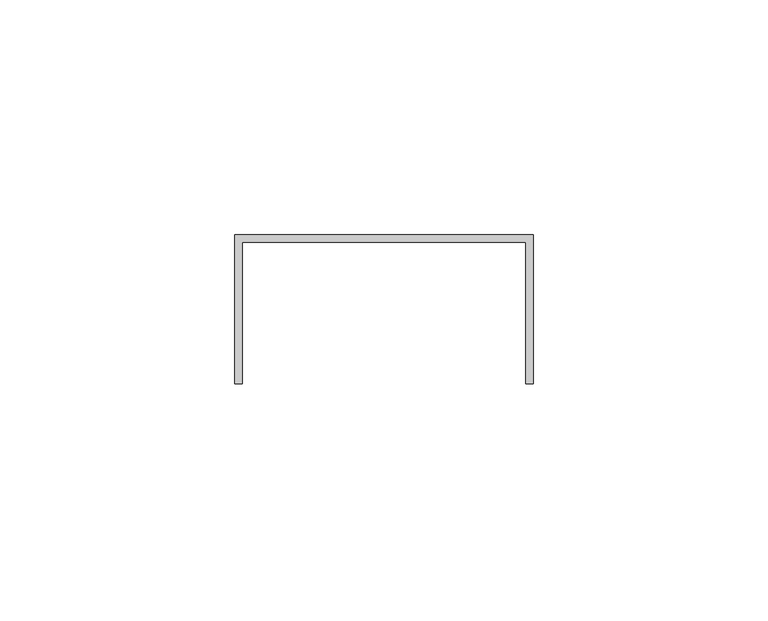
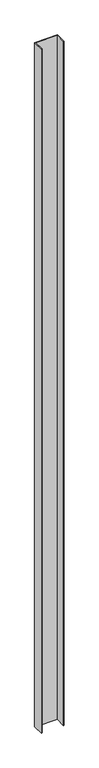
"""IFC4 building model written with IfcOpenShell, lengths in millimetres: proxy geometry, Generic Models 7:Generic Models 1:3:Generic Models 1:3 : Generic Models 7:Generic Models 1:305549:3:Generic Models 1:3:Generic Models 1:3 : Generic Models 7:Generic Models 1:305549:3 : Generic Models 7:Generic Models 1:3:Generic Models 1:3 : Generic Models 7:Generic Models 1:305549:301244:23 : Generic Models 7:Generic Models 1:3:Generic Models 1:3 : Generic Models 7:Generic Models 1:305549:3:Generic Models 1:3:Generic Models 1:3 : Generic Models 7:Generic Models 1:305549:3 : Generic Models 7:Generic Models 1:3:Generic Models 1:3 : Generic Models 7:Generic Models 1:305549:301244:308848."""

from ifc_helpers import new_model, si_unit, frame, origin, place, context, project, spatial, polyline, outline, extrude, source, transform, mapped, element, save


def generic_models_0d41abfa(model_context):
    return source(origin(), model_context, "Body", "SweptSolid", [
        extrude(outline(polyline([(579320.411724, -578742.9707955), (579383.9117239, -578742.9707955), (579383.9117239, -578774.7207955), (579382.3242239, -578774.7207955), (579382.3242239, -578744.5582955), (579321.999224, -578744.5582955), (579321.999224, -578774.7207955), (579320.411724, -578774.7207955), (579320.411724, -578742.9707955)])), frame((0.0, 0.0, 4133.81326), z_axis=(0.0, 0.0, 1.0), x_axis=(1.0, 0.0, 0.0)), (0.0, 0.0, 1.0), 2000.28674),
    ])


if __name__ == "__main__":
    model = new_model("IFC4")
    model_context = context("Model", 3, world=origin())
    ifc_project = project(units=[si_unit("LENGTHUNIT", "METRE", prefix="MILLI")], contexts=[model_context])
    site = spatial("IfcSite", under=ifc_project)
    building = spatial("IfcBuilding", under=site)
    placement = place(None, origin())
    generic_models_shape = generic_models_0d41abfa(model_context)
    element("IfcBuildingElementProxy", 1, Name="Generic Models 7:Generic Models 1:3:Generic Models 1:3 : Generic Models 7:Generic Models 1:305549:3:Generic Models 1:3:Generic Models 1:3 : Generic Models 7:Generic Models 1:305549:3 : Generic Models 7:Generic Models 1:3:Generic Models 1:3 : Generic Models 7:Generic Models 1:305549:301244:23 : Generic Models 7:Generic Models 1:3:Generic Models 1:3 : Generic Models 7:Generic Models 1:305549:3:Generic Models 1:3:Generic Models 1:3 : Generic Models 7:Generic Models 1:305549:3 : Generic Models 7:Generic Models 1:3:Generic Models 1:3 : Generic Models 7:Generic Models 1:305549:301244:308848", ObjectType="Generic Models 7:Generic Models 1:3:Generic Models 1:3 : Generic Models 7:Generic Models 1:305549:3:Generic Models 1:3:Generic Models 1:3 : Generic Models 7:Generic Models 1:305549:3 : Generic Models 7:Generic Models 1:3:Generic Models 1:3 : Generic Models 7:Generic Models 1:305549:301244:23 : Generic Models 7:Generic Models 1:3:Generic Models 1:3 : Generic Models 7:Generic Models 1:305549:3:Generic Models 1:3:Generic Models 1:3 : Generic Models 7:Generic Models 1:305549:3 : Generic Models 7:Generic Models 1:3:Generic Models 1:3 : Generic Models 7:Generic Models 1:305549:301244:308848", at=placement, inside=building, context=model_context, shape_type="MappedRepresentation", body=[
        mapped(generic_models_shape, transform((0.0, 0.0, 0.0), x_axis=(1.0, 0.0, 0.0), y_axis=(0.0, 1.0, 0.0), z_axis=(0.0, 0.0, 1.0))),
    ])
    save(model, "model.ifc")

# Revit data of these elements
# Type "Generic Models 7:Generic Models 1:3:Generic Models 1:3 : Generic Models 7:Generic Models 1:305549:3:Generic Models 1:3:Generic Models 1:3 : Generic Models 7:Generic Models 1:305549:3 : Generic Models 7:Generic Models 1:3:Generic Models 1:3 : Generic Models 7:Generic Models 1:305549:301244:23 : Generic Models 7:Generic Models 1:3:Generic Models 1:3 : Generic Models 7:Generic Models 1:305549:3:Generic Models 1:3:Generic Models 1:3 : Generic Models 7:Generic Models 1:305549:3 : Generic Models 7:Generic Models 1:3:Generic Models 1:3 : Generic Models 7:Generic Models 1:305549:301244:308848"
#   NameOverride = "Generic Models 7:Generic Models 1:3:Generic Models 1:3 : Generic Models 7:Generic Models 1:305549:3:Generic Models 1:3:Generic Models 1:3 : Generic Models 7:Generic Models 1:305549:3 : Generic Models 7:Generic Models 1:3:Generic Models 1:3 : Generic Models 7:Generic Models 1:305549:301244:308848"
#   ObjectTypeOverride = "Generic Models 1:3:Generic Models 1:3 : Generic Models 7:Generic Models 1:305549:3 : Generic Models 7:Generic Models 1:3:Generic Models 1:3 : Generic Models 7:Generic Models 1:305549:301244"
#   Reference = "Generic Models 1"
#   Tag = "308848"
# Element 1 (IfcBuildingElementProxy, "Generic Models 7:Generic Models 1:3:Generic Models 1:3 : Generic Models 7:Generic Models 1:305549:3:Generic Models 1:3:Generic Models 1:3 : Generic Models 7:Generic Models 1:305549:3 : Generic Models 7:Generic Models 1:3:Generic Models 1:3 : Generic Models 7:Generic Models 1:305549:301244:23 : Generic Models 7:Generic Models 1:3:Generic Models 1:3 : Generic Models 7:Generic Models 1:305549:3:Generic Models 1:3:Generic Models 1:3 : Generic Models 7:Generic Models 1:305549:3 : Generic Models 7:Generic Models 1:3:Generic Models 1:3 : Generic Models 7:Generic Models 1:305549:301244:308848")
#   Materials on its faces: "GALVANIZED U-CHANNEL (250T125-33)"
# Materials
#   "GALVANIZED U-CHANNEL (250T125-33)": class "Unassigned", colour RGB 202 201 200, transparency 0, Keynote = "M05451300.02", Cost = 0
